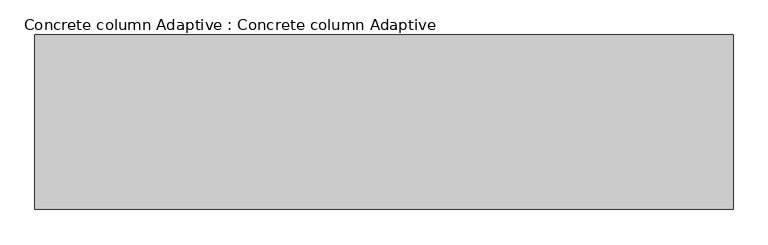
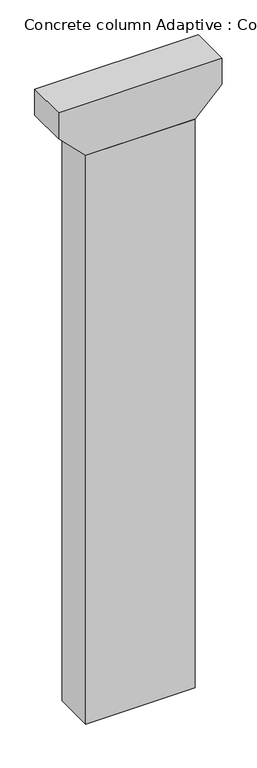
"""IFC4 building model written with IfcOpenShell, lengths in millimetres: proxy geometry, Concrete column Adaptive : Concrete column Adaptive."""

from ifc_helpers import new_model, si_unit, frame, origin, origin_with_axes, place, context, project, spatial, polyline, outline, extrude, source, transform, mapped, element, save


def concrete_column_adaptive_concrete_column_adaptive_2f6c8aee(model_context):
    return source(origin(), model_context, "Body", "SweptSolid", [
        extrude(outline(polyline([(48034.0, 6000.0), (48034.0, -6000.0), (46034.0, -6000.0), (44034.0, -4000.0), (44034.0, 4000.0), (46034.0, 6000.0), (48034.0, 6000.0)])), frame((0.0, -1500.0, 0.0), z_axis=(0.0, 1.0, 0.0), x_axis=(0.0, 0.0, 1.0)), (0.0, 0.0, 1.0), 3000.0),
        extrude(outline(polyline([(-4000.0, -1500.0), (-4000.0, 1500.0), (4000.0, 1500.0), (4000.0, -1500.0), (-4000.0, -1500.0)])), origin_with_axes(), (0.0, 0.0, 1.0), 44034.0),
    ])


if __name__ == "__main__":
    model = new_model("IFC4")
    model_context = context("Model", 3, world=origin())
    ifc_project = project(units=[si_unit("LENGTHUNIT", "METRE", prefix="MILLI")], contexts=[model_context])
    site = spatial("IfcSite", under=ifc_project)
    building = spatial("IfcBuilding", under=site)
    placement = place(None, origin())
    concrete_column_adaptive_concrete_column_adaptive_shape = concrete_column_adaptive_concrete_column_adaptive_2f6c8aee(model_context)
    element("IfcBuildingElementProxy", 1, Name="Concrete column Adaptive : Concrete column Adaptive", ObjectType="Concrete column Adaptive : Concrete column Adaptive", at=placement, inside=building, context=model_context, shape_type="MappedRepresentation", body=[
        mapped(concrete_column_adaptive_concrete_column_adaptive_shape, transform((0.0, 0.0, 0.0), x_axis=(1.0, 0.0, 0.0), y_axis=(0.0, 1.0, 0.0), z_axis=(0.0, 0.0, 1.0))),
    ])
    save(model, "model.ifc")

# Revit data of these elements
# Type "Concrete column Adaptive : Concrete column Adaptive"
#   Height [instance default] = 30000 mm
#   Default Elevation = 0
# Element 1 (IfcBuildingElementProxy, "Concrete column Adaptive : Concrete column Adaptive")
#   Height = 44034 mm
